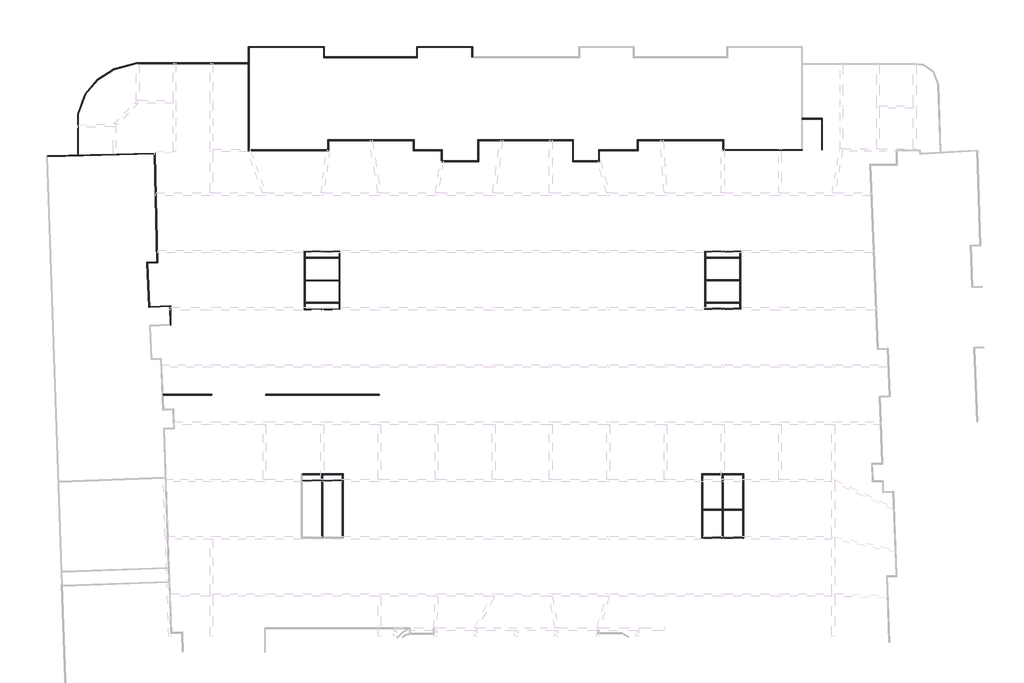
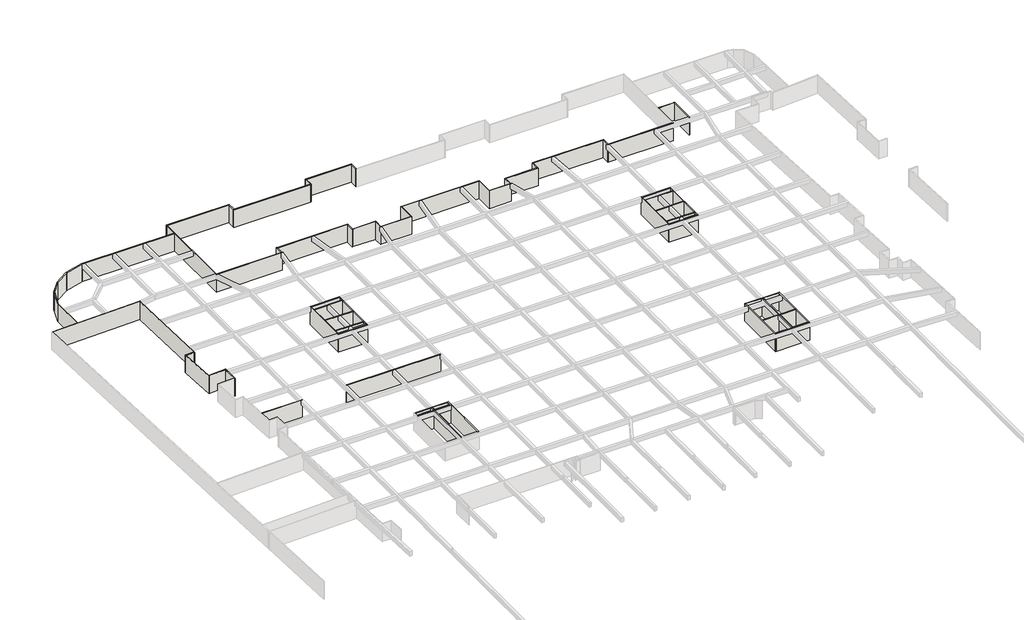
# One storey, part 3 of 8: 64 walls.
"""IFC4 building model written with IfcOpenShell, lengths in millimetres."""

from ifc_helpers import new_model, si_unit, origin, origin_with_axes, place, context, project, spatial, polyline, outline, extrude, faceted_brep, element, save

model = new_model("IFC4")

# Units and contexts
model_context = context("Model", 3, world=origin())
ifc_project = project(units=[si_unit("LENGTHUNIT", "METRE", prefix="MILLI")], contexts=[model_context])

# Site, building, storey
site = spatial("IfcSite", under=ifc_project)
building = spatial("IfcBuilding", under=site)
storey = spatial("IfcBuildingStorey", under=building, Name="户型图", Elevation=0.0)

# Walls
placement = place(None, origin())
element("IfcWall", 1, ObjectType="所有墙体", at=placement, inside=storey, context=model_context, shape_type="Brep", body=[
    faceted_brep([(652720.3094441, -903322.0093989, 0.0), (668403.5865909, -902923.6273505, 0.0), (668523.5478948, -902920.5801283, 0.0), (668523.5478948, -902920.5801283, 3300.0), (668403.5865909, -902923.6273505, 3300.0), (652720.3094441, -903322.0093989, 3300.0), (652716.1213151, -903202.077076, 0.0), (652716.1213151, -903202.077076, 3300.0), (657153.6402454, -903089.3565097, 3300.0), (657273.6402454, -903086.3083045, 3300.0), (668520.5006726, -902800.6188244, 3300.0), (668520.5006726, -902800.6188244, 0.0), (657273.6402454, -903086.3083045, 0.0), (657153.6402454, -903089.3565097, 0.0)], [[[0, 1, 2, 3, 4, 5]], [[6, 7, 8, 9, 10, 11, 12, 13]], [[2, 1, 0, 6, 13, 12, 11]], [[5, 4, 3, 10, 9, 8, 7]], [[0, 5, 7, 6]], [[3, 2, 11, 10]]]),
])
element("IfcWall", 2, ObjectType="所有墙体", at=placement, inside=storey, context=model_context, shape_type="Brep", body=[
    faceted_brep([(668403.5865909, -902923.6273505, 0.0), (668806.8356594, -918798.5065686, 0.0), (668809.8828816, -918918.4678725, 0.0), (668809.8828816, -918918.4678725, 3300.0), (668806.8356594, -918798.5065686, 3300.0), (668403.5865909, -902923.6273505, 3300.0), (668523.5478948, -902920.5801283, 0.0), (668523.5478948, -902920.5801283, 3300.0), (668929.8441855, -918915.4206503, 3300.0), (668929.8441855, -918915.4206503, 0.0)], [[[0, 1, 2, 3, 4, 5]], [[6, 7, 8, 9]], [[2, 1, 0, 6, 9]], [[5, 4, 3, 8, 7]], [[0, 5, 7, 6]], [[3, 2, 9, 8]]]),
])
element("IfcWall", 3, ObjectType="所有墙体", at=placement, inside=storey, context=model_context, shape_type="Brep", body=[
    faceted_brep([(668806.8356594, -918798.5065686, 0.0), (667306.1591427, -918836.6263174, 0.0), (667306.1591427, -918836.6263174, 3300.0), (668806.8356594, -918798.5065686, 3300.0), (668809.8828816, -918918.4678725, 0.0), (668809.8828816, -918918.4678725, 3300.0), (667431.4881043, -918953.4814561, 3300.0), (667311.504784, -918956.5292375, 3300.0), (667311.504784, -918956.5292375, 0.0), (667431.4881043, -918953.4814561, 0.0)], [[[0, 1, 2, 3]], [[4, 5, 6, 7, 8, 9]], [[1, 0, 4, 9, 8]], [[3, 2, 7, 6, 5]], [[0, 3, 5, 4]], [[2, 1, 8, 7]]]),
])
element("IfcWall", 4, ObjectType="所有墙体", at=placement, inside=storey, context=model_context, shape_type="Brep", body=[
    faceted_brep([(667311.504784, -918956.5292375, 0.0), (667601.6118634, -925463.6411151, 0.0), (667601.6118634, -925463.6411151, 3300.0), (667311.504784, -918956.5292375, 3300.0), (667431.4881043, -918953.4814561, 0.0), (667431.4881043, -918953.4814561, 3300.0), (667716.1481214, -925338.4155362, 3300.0), (667721.4927818, -925458.2964547, 3300.0), (667721.4927818, -925458.2964547, 0.0), (667716.1481214, -925338.4155362, 0.0)], [[[0, 1, 2, 3]], [[4, 5, 6, 7, 8, 9]], [[1, 0, 4, 9, 8]], [[3, 2, 7, 6, 5]], [[0, 3, 5, 4]], [[2, 1, 8, 7]]]),
])
element("IfcWall", 5, ObjectType="所有墙体", at=placement, inside=storey, context=model_context, shape_type="Brep", body=[
    faceted_brep([(667721.4927818, -925458.2964547, 0.0), (670697.0897488, -925325.6351816, 0.0), (670817.0147025, -925320.288558, 0.0), (670817.0147025, -925320.288558, 3300.0), (670697.0897488, -925325.6351816, 3300.0), (667721.4927818, -925458.2964547, 3300.0), (667716.1481214, -925338.4155362, 0.0), (667716.1481214, -925338.4155362, 3300.0), (670814.9196444, -925200.2627623, 3300.0), (670814.9196444, -925200.2627623, 0.0)], [[[0, 1, 2, 3, 4, 5]], [[6, 7, 8, 9]], [[2, 1, 0, 6, 9]], [[5, 4, 3, 8, 7]], [[0, 5, 7, 6]], [[3, 2, 9, 8]]]),
])
element("IfcWall", 6, ObjectType="所有墙体", at=placement, inside=storey, context=model_context, shape_type="Brep", body=[
    faceted_brep([(670697.0897488, -925325.6351816, 0.0), (670742.7384573, -927940.8479412, 0.0), (670744.8335153, -928060.8737369, 0.0), (670744.8335153, -928060.8737369, 3300.0), (670742.7384573, -927940.8479412, 3300.0), (670697.0897488, -925325.6351816, 3300.0), (670817.0147025, -925320.288558, 0.0), (670817.0147025, -925320.288558, 3300.0), (670864.758469, -928055.5271133, 3300.0), (670864.758469, -928055.5271133, 0.0)], [[[0, 1, 2, 3, 4, 5]], [[6, 7, 8, 9]], [[2, 1, 0, 6, 9]], [[5, 4, 3, 8, 7]], [[0, 5, 7, 6]], [[3, 2, 9, 8]]]),
])
element("IfcWall", 7, ObjectType="所有墙体", at=placement, inside=storey, context=model_context, shape_type="Brep", body=[
    faceted_brep([(766494.1555611, -902351.7569482, 0.0), (766494.1555611, -897691.7569482, 0.0), (766494.1555611, -897691.7569482, 3300.0), (766494.1555611, -902351.7569482, 3300.0), (766374.1555611, -902351.7569482, 0.0), (766374.1555611, -902351.7569482, 3300.0), (766374.1555611, -897811.7569482, 3300.0), (766374.1555611, -897691.7569482, 3300.0), (766374.1555611, -897691.7569482, 0.0), (766374.1555611, -897811.7569482, 0.0)], [[[0, 1, 2, 3]], [[4, 5, 6, 7, 8, 9]], [[1, 0, 4, 9, 8]], [[3, 2, 7, 6, 5]], [[0, 3, 5, 4]], [[2, 1, 8, 7]]]),
])
element("IfcWall", 8, ObjectType="所有墙体", at=placement, inside=storey, context=model_context, shape_type="SweptSolid", body=[
    extrude(outline(polyline([(763544.1555611, -897691.7569482), (766374.1555611, -897691.7569482), (766374.1555611, -897811.7569482), (763544.1555611, -897811.7569482), (763544.1555611, -897691.7569482)])), origin_with_axes(), (0.0, 0.0, 1.0), 3300.0),
])
element("IfcWall", 9, ObjectType="所有墙体", at=placement, inside=storey, context=model_context, shape_type="Brep", body=[
    faceted_brep([(715144.1555611, -888666.7569482, 0.0), (715144.1555611, -887166.8168633, 0.0), (715144.1555611, -887166.8168633, 3300.0), (715144.1555611, -888666.7569482, 3300.0), (715024.1555611, -888666.7569482, 0.0), (715024.1555611, -888666.7569482, 3300.0), (715024.1555611, -887286.8168633, 3300.0), (715024.1555611, -887166.8168633, 3300.0), (715024.1555611, -887166.8168633, 0.0), (715024.1555611, -887286.8168633, 0.0)], [[[0, 1, 2, 3]], [[4, 5, 6, 7, 8, 9]], [[1, 0, 4, 9, 8]], [[3, 2, 7, 6, 5]], [[0, 3, 5, 4]], [[2, 1, 8, 7]]]),
])
element("IfcWall", 10, ObjectType="所有墙体", at=placement, inside=storey, context=model_context, shape_type="Brep", body=[
    faceted_brep([(715024.1555611, -887166.8168633, 0.0), (706904.1555611, -887166.8168633, 0.0), (706904.1555611, -887166.8168633, 3300.0), (715024.1555611, -887166.8168633, 3300.0), (715024.1555611, -887286.8168633, 0.0), (715024.1555611, -887286.8168633, 3300.0), (707024.1555611, -887286.8168633, 3300.0), (706904.1555611, -887286.8168633, 3300.0), (706904.1555611, -887286.8168633, 0.0), (707024.1555611, -887286.8168633, 0.0)], [[[0, 1, 2, 3]], [[4, 5, 6, 7, 8, 9]], [[1, 0, 4, 9, 8]], [[3, 2, 7, 6, 5]], [[0, 3, 5, 4]], [[2, 1, 8, 7]]]),
])
element("IfcWall", 11, ObjectType="所有墙体", at=placement, inside=storey, context=model_context, shape_type="Brep", body=[
    faceted_brep([(706904.1555611, -887286.8168633, 0.0), (706904.1555611, -888666.7569482, 0.0), (706904.1555611, -888786.7569482, 0.0), (706904.1555611, -888786.7569482, 3300.0), (706904.1555611, -888666.7569482, 3300.0), (706904.1555611, -887286.8168633, 3300.0), (707024.1555611, -887286.8168633, 0.0), (707024.1555611, -887286.8168633, 3300.0), (707024.1555611, -888786.7569482, 3300.0), (707024.1555611, -888786.7569482, 0.0)], [[[0, 1, 2, 3, 4, 5]], [[6, 7, 8, 9]], [[2, 1, 0, 6, 9]], [[5, 4, 3, 8, 7]], [[0, 5, 7, 6]], [[3, 2, 9, 8]]]),
])
element("IfcWall", 12, ObjectType="所有墙体", at=placement, inside=storey, context=model_context, shape_type="Brep", body=[
    faceted_brep([(706904.1555611, -888666.7569482, 0.0), (693394.1555611, -888666.7569482, 0.0), (693274.1555611, -888666.7569482, 0.0), (693274.1555611, -888666.7569482, 3300.0), (693394.1555611, -888666.7569482, 3300.0), (706904.1555611, -888666.7569482, 3300.0), (706904.1555611, -888786.7569482, 0.0), (706904.1555611, -888786.7569482, 3300.0), (693274.1555611, -888786.7569482, 3300.0), (693274.1555611, -888786.7569482, 0.0)], [[[0, 1, 2, 3, 4, 5]], [[6, 7, 8, 9]], [[2, 1, 0, 6, 9]], [[5, 4, 3, 8, 7]], [[0, 5, 7, 6]], [[3, 2, 9, 8]]]),
])
element("IfcWall", 13, ObjectType="所有墙体", at=placement, inside=storey, context=model_context, shape_type="Brep", body=[
    faceted_brep([(693394.1555611, -888666.7569482, 0.0), (693394.1555611, -887166.8168633, 0.0), (693394.1555611, -887166.8168633, 3300.0), (693394.1555611, -888666.7569482, 3300.0), (693274.1555611, -888666.7569482, 0.0), (693274.1555611, -888666.7569482, 3300.0), (693274.1555611, -887286.8168633, 3300.0), (693274.1555611, -887166.8168633, 3300.0), (693274.1555611, -887166.8168633, 0.0), (693274.1555611, -887286.8168633, 0.0)], [[[0, 1, 2, 3]], [[4, 5, 6, 7, 8, 9]], [[1, 0, 4, 9, 8]], [[3, 2, 7, 6, 5]], [[0, 3, 5, 4]], [[2, 1, 8, 7]]]),
])
element("IfcWall", 14, ObjectType="所有墙体", at=placement, inside=storey, context=model_context, shape_type="Brep", body=[
    faceted_brep([(693274.1555611, -887166.8168633, 0.0), (682227.1185384, -887166.8168633, 0.0), (682227.1185384, -887166.8168633, 3300.0), (693274.1555611, -887166.8168633, 3300.0), (693274.1555611, -887286.8168633, 0.0), (693274.1555611, -887286.8168633, 3300.0), (682347.1185384, -887286.8168633, 3300.0), (682227.1185384, -887286.8168633, 3300.0), (682227.1185384, -887286.8168633, 0.0), (682347.1185384, -887286.8168633, 0.0)], [[[0, 1, 2, 3]], [[4, 5, 6, 7, 8, 9]], [[1, 0, 4, 9, 8]], [[3, 2, 7, 6, 5]], [[0, 3, 5, 4]], [[2, 1, 8, 7]]]),
])
element("IfcWall", 15, ObjectType="所有墙体", at=placement, inside=storey, context=model_context, shape_type="Brep", body=[
    faceted_brep([(682227.1185384, -887286.8168633, 0.0), (682227.1185384, -889568.8408137, 0.0), (682227.1185384, -889688.8408137, 0.0), (682227.1185384, -902461.3967018, 0.0), (682227.1185384, -902461.3967018, 3300.0), (682227.1185384, -889688.8408137, 3300.0), (682227.1185384, -889568.8408137, 3300.0), (682227.1185384, -887286.8168633, 3300.0), (682347.1185384, -887286.8168633, 0.0), (682347.1185384, -887286.8168633, 3300.0), (682347.1185384, -902341.3967018, 3300.0), (682347.1185384, -902461.3967018, 3300.0), (682347.1185384, -902461.3967018, 0.0), (682347.1185384, -902341.3967018, 0.0)], [[[0, 1, 2, 3, 4, 5, 6, 7]], [[8, 9, 10, 11, 12, 13]], [[3, 2, 1, 0, 8, 13, 12]], [[7, 6, 5, 4, 11, 10, 9]], [[0, 7, 9, 8]], [[4, 3, 12, 11]]]),
])
element("IfcWall", 16, ObjectType="所有墙体", at=placement, inside=storey, context=model_context, shape_type="Brep", body=[
    faceted_brep([(682347.1185384, -902461.3967018, 0.0), (693994.1555611, -902461.3967018, 0.0), (693994.1555611, -902461.3967018, 3300.0), (682347.1185384, -902461.3967018, 3300.0), (682347.1185384, -902341.3967018, 0.0), (682347.1185384, -902341.3967018, 3300.0), (693874.1555611, -902341.3967018, 3300.0), (693994.1555611, -902341.3967018, 3300.0), (693994.1555611, -902341.3967018, 0.0), (693874.1555611, -902341.3967018, 0.0)], [[[0, 1, 2, 3]], [[4, 5, 6, 7, 8, 9]], [[1, 0, 4, 9, 8]], [[3, 2, 7, 6, 5]], [[0, 3, 5, 4]], [[2, 1, 8, 7]]]),
])
element("IfcWall", 17, ObjectType="所有墙体", at=placement, inside=storey, context=model_context, shape_type="Brep", body=[
    faceted_brep([(693994.1555611, -902341.3967018, 0.0), (693994.1555611, -900986.7569482, 0.0), (693994.1555611, -900866.7569482, 0.0), (693994.1555611, -900866.7569482, 3300.0), (693994.1555611, -900986.7569482, 3300.0), (693994.1555611, -902341.3967018, 3300.0), (693874.1555611, -902341.3967018, 0.0), (693874.1555611, -902341.3967018, 3300.0), (693874.1555611, -900866.7569482, 3300.0), (693874.1555611, -900866.7569482, 0.0)], [[[0, 1, 2, 3, 4, 5]], [[6, 7, 8, 9]], [[2, 1, 0, 6, 9]], [[5, 4, 3, 8, 7]], [[0, 5, 7, 6]], [[3, 2, 9, 8]]]),
])
element("IfcWall", 18, ObjectType="所有墙体", at=placement, inside=storey, context=model_context, shape_type="Brep", body=[
    faceted_brep([(693994.1555611, -900986.7569482, 0.0), (706424.1555611, -900986.7569482, 0.0), (706544.1555611, -900986.7569482, 0.0), (706544.1555611, -900986.7569482, 3300.0), (706424.1555611, -900986.7569482, 3300.0), (693994.1555611, -900986.7569482, 3300.0), (693994.1555611, -900866.7569482, 0.0), (693994.1555611, -900866.7569482, 3300.0), (706544.1555611, -900866.7569482, 3300.0), (706544.1555611, -900866.7569482, 0.0)], [[[0, 1, 2, 3, 4, 5]], [[6, 7, 8, 9]], [[2, 1, 0, 6, 9]], [[5, 4, 3, 8, 7]], [[0, 5, 7, 6]], [[3, 2, 9, 8]]]),
])
element("IfcWall", 19, ObjectType="所有墙体", at=placement, inside=storey, context=model_context, shape_type="Brep", body=[
    faceted_brep([(706424.1555611, -900986.7569482, 0.0), (706424.1555611, -902461.3967018, 0.0), (706424.1555611, -902461.3967018, 3300.0), (706424.1555611, -900986.7569482, 3300.0), (706544.1555611, -900986.7569482, 0.0), (706544.1555611, -900986.7569482, 3300.0), (706544.1555611, -902341.3967018, 3300.0), (706544.1555611, -902461.3967018, 3300.0), (706544.1555611, -902461.3967018, 0.0), (706544.1555611, -902341.3967018, 0.0)], [[[0, 1, 2, 3]], [[4, 5, 6, 7, 8, 9]], [[1, 0, 4, 9, 8]], [[3, 2, 7, 6, 5]], [[0, 3, 5, 4]], [[2, 1, 8, 7]]]),
])
element("IfcWall", 20, ObjectType="所有墙体", at=placement, inside=storey, context=model_context, shape_type="Brep", body=[
    faceted_brep([(706544.1555611, -902461.3967018, 0.0), (710546.3042159, -902461.3967018, 0.0), (710666.3042159, -902461.3967018, 0.0), (710666.3042159, -902461.3967018, 3300.0), (710546.3042159, -902461.3967018, 3300.0), (706544.1555611, -902461.3967018, 3300.0), (706544.1555611, -902341.3967018, 0.0), (706544.1555611, -902341.3967018, 3300.0), (710666.3042159, -902341.3967018, 3300.0), (710666.3042159, -902341.3967018, 0.0)], [[[0, 1, 2, 3, 4, 5]], [[6, 7, 8, 9]], [[2, 1, 0, 6, 9]], [[5, 4, 3, 8, 7]], [[0, 5, 7, 6]], [[3, 2, 9, 8]]]),
])
element("IfcWall", 21, ObjectType="所有墙体", at=placement, inside=storey, context=model_context, shape_type="Brep", body=[
    faceted_brep([(710546.3042159, -902461.3967018, 0.0), (710546.3042159, -904061.7569482, 0.0), (710546.3042159, -904061.7569482, 3300.0), (710546.3042159, -902461.3967018, 3300.0), (710666.3042159, -902461.3967018, 0.0), (710666.3042159, -902461.3967018, 3300.0), (710666.3042159, -903941.7569482, 3300.0), (710666.3042159, -904061.7569482, 3300.0), (710666.3042159, -904061.7569482, 0.0), (710666.3042159, -903941.7569482, 0.0)], [[[0, 1, 2, 3]], [[4, 5, 6, 7, 8, 9]], [[1, 0, 4, 9, 8]], [[3, 2, 7, 6, 5]], [[0, 3, 5, 4]], [[2, 1, 8, 7]]]),
])
element("IfcWall", 22, ObjectType="所有墙体", at=placement, inside=storey, context=model_context, shape_type="Brep", body=[
    faceted_brep([(710666.3042159, -904061.7569482, 0.0), (716044.1555611, -904061.7569482, 0.0), (716044.1555611, -904061.7569482, 3300.0), (710666.3042159, -904061.7569482, 3300.0), (710666.3042159, -903941.7569482, 0.0), (710666.3042159, -903941.7569482, 3300.0), (715924.1555611, -903941.7569482, 3300.0), (716044.1555611, -903941.7569482, 3300.0), (716044.1555611, -903941.7569482, 0.0), (715924.1555611, -903941.7569482, 0.0)], [[[0, 1, 2, 3]], [[4, 5, 6, 7, 8, 9]], [[1, 0, 4, 9, 8]], [[3, 2, 7, 6, 5]], [[0, 3, 5, 4]], [[2, 1, 8, 7]]]),
])
element("IfcWall", 23, ObjectType="所有墙体", at=placement, inside=storey, context=model_context, shape_type="Brep", body=[
    faceted_brep([(716044.1555611, -903941.7569482, 0.0), (716044.1555611, -900986.7569482, 0.0), (716044.1555611, -900866.7569482, 0.0), (716044.1555611, -900866.7569482, 3300.0), (716044.1555611, -900986.7569482, 3300.0), (716044.1555611, -903941.7569482, 3300.0), (715924.1555611, -903941.7569482, 0.0), (715924.1555611, -903941.7569482, 3300.0), (715924.1555611, -900866.7569482, 3300.0), (715924.1555611, -900866.7569482, 0.0)], [[[0, 1, 2, 3, 4, 5]], [[6, 7, 8, 9]], [[2, 1, 0, 6, 9]], [[5, 4, 3, 8, 7]], [[0, 5, 7, 6]], [[3, 2, 9, 8]]]),
])
element("IfcWall", 24, ObjectType="所有墙体", at=placement, inside=storey, context=model_context, shape_type="Brep", body=[
    faceted_brep([(716044.1555611, -900986.7569482, 0.0), (729824.1555611, -900986.7569482, 0.0), (729944.1555611, -900986.7569482, 0.0), (729944.1555611, -900986.7569482, 3300.0), (729824.1555611, -900986.7569482, 3300.0), (716044.1555611, -900986.7569482, 3300.0), (716044.1555611, -900866.7569482, 0.0), (716044.1555611, -900866.7569482, 3300.0), (729944.1555611, -900866.7569482, 3300.0), (729944.1555611, -900866.7569482, 0.0)], [[[0, 1, 2, 3, 4, 5]], [[6, 7, 8, 9]], [[2, 1, 0, 6, 9]], [[5, 4, 3, 8, 7]], [[0, 5, 7, 6]], [[3, 2, 9, 8]]]),
])
element("IfcWall", 25, ObjectType="所有墙体", at=placement, inside=storey, context=model_context, shape_type="Brep", body=[
    faceted_brep([(729824.1555611, -900986.7569482, 0.0), (729824.1555611, -904061.7569482, 0.0), (729824.1555611, -904061.7569482, 3300.0), (729824.1555611, -900986.7569482, 3300.0), (729944.1555611, -900986.7569482, 0.0), (729944.1555611, -900986.7569482, 3300.0), (729944.1555611, -903941.7569482, 3300.0), (729944.1555611, -904061.7569482, 3300.0), (729944.1555611, -904061.7569482, 0.0), (729944.1555611, -903941.7569482, 0.0)], [[[0, 1, 2, 3]], [[4, 5, 6, 7, 8, 9]], [[1, 0, 4, 9, 8]], [[3, 2, 7, 6, 5]], [[0, 3, 5, 4]], [[2, 1, 8, 7]]]),
])
element("IfcWall", 26, ObjectType="所有墙体", at=placement, inside=storey, context=model_context, shape_type="Brep", body=[
    faceted_brep([(729944.1555611, -904061.7569482, 0.0), (733744.1555611, -904061.7569482, 0.0), (733744.1555611, -904061.7569482, 3300.0), (729944.1555611, -904061.7569482, 3300.0), (729944.1555611, -903941.7569482, 0.0), (729944.1555611, -903941.7569482, 3300.0), (733624.1555611, -903941.7569482, 3300.0), (733744.1555611, -903941.7569482, 3300.0), (733744.1555611, -903941.7569482, 0.0), (733624.1555611, -903941.7569482, 0.0)], [[[0, 1, 2, 3]], [[4, 5, 6, 7, 8, 9]], [[1, 0, 4, 9, 8]], [[3, 2, 7, 6, 5]], [[0, 3, 5, 4]], [[2, 1, 8, 7]]]),
])
element("IfcWall", 27, ObjectType="所有墙体", at=placement, inside=storey, context=model_context, shape_type="Brep", body=[
    faceted_brep([(733744.1555611, -903941.7569482, 0.0), (733744.1555611, -902461.3967018, 0.0), (733744.1555611, -902341.3967018, 0.0), (733744.1555611, -902341.3967018, 3300.0), (733744.1555611, -902461.3967018, 3300.0), (733744.1555611, -903941.7569482, 3300.0), (733624.1555611, -903941.7569482, 0.0), (733624.1555611, -903941.7569482, 3300.0), (733624.1555611, -902341.3967018, 3300.0), (733624.1555611, -902341.3967018, 0.0)], [[[0, 1, 2, 3, 4, 5]], [[6, 7, 8, 9]], [[2, 1, 0, 6, 9]], [[5, 4, 3, 8, 7]], [[0, 5, 7, 6]], [[3, 2, 9, 8]]]),
])
element("IfcWall", 28, ObjectType="所有墙体", at=placement, inside=storey, context=model_context, shape_type="Brep", body=[
    faceted_brep([(733744.1555611, -902461.3967018, 0.0), (739444.1555611, -902461.3967018, 0.0), (739444.1555611, -902461.3967018, 3300.0), (733744.1555611, -902461.3967018, 3300.0), (733744.1555611, -902341.3967018, 0.0), (733744.1555611, -902341.3967018, 3300.0), (739324.1555611, -902341.3967018, 3300.0), (739444.1555611, -902341.3967018, 3300.0), (739444.1555611, -902341.3967018, 0.0), (739324.1555611, -902341.3967018, 0.0)], [[[0, 1, 2, 3]], [[4, 5, 6, 7, 8, 9]], [[1, 0, 4, 9, 8]], [[3, 2, 7, 6, 5]], [[0, 3, 5, 4]], [[2, 1, 8, 7]]]),
])
element("IfcWall", 29, ObjectType="所有墙体", at=placement, inside=storey, context=model_context, shape_type="Brep", body=[
    faceted_brep([(739444.1555611, -902341.3967018, 0.0), (739444.1555611, -900986.7569482, 0.0), (739444.1555611, -900866.7569482, 0.0), (739444.1555611, -900866.7569482, 3300.0), (739444.1555611, -900986.7569482, 3300.0), (739444.1555611, -902341.3967018, 3300.0), (739324.1555611, -902341.3967018, 0.0), (739324.1555611, -902341.3967018, 3300.0), (739324.1555611, -900866.7569482, 3300.0), (739324.1555611, -900866.7569482, 0.0)], [[[0, 1, 2, 3, 4, 5]], [[6, 7, 8, 9]], [[2, 1, 0, 6, 9]], [[5, 4, 3, 8, 7]], [[0, 5, 7, 6]], [[3, 2, 9, 8]]]),
])
element("IfcWall", 30, ObjectType="所有墙体", at=placement, inside=storey, context=model_context, shape_type="Brep", body=[
    faceted_brep([(739444.1555611, -900986.7569482, 0.0), (751874.1555611, -900986.7569482, 0.0), (751994.1555611, -900986.7569482, 0.0), (751994.1555611, -900986.7569482, 3300.0), (751874.1555611, -900986.7569482, 3300.0), (739444.1555611, -900986.7569482, 3300.0), (739444.1555611, -900866.7569482, 0.0), (739444.1555611, -900866.7569482, 3300.0), (751994.1555611, -900866.7569482, 3300.0), (751994.1555611, -900866.7569482, 0.0)], [[[0, 1, 2, 3, 4, 5]], [[6, 7, 8, 9]], [[2, 1, 0, 6, 9]], [[5, 4, 3, 8, 7]], [[0, 5, 7, 6]], [[3, 2, 9, 8]]]),
])
element("IfcWall", 31, ObjectType="所有墙体", at=placement, inside=storey, context=model_context, shape_type="Brep", body=[
    faceted_brep([(751874.1555611, -900986.7569482, 0.0), (751874.1555611, -902411.7569482, 0.0), (751874.1555611, -902411.7569482, 3300.0), (751874.1555611, -900986.7569482, 3300.0), (751994.1555611, -900986.7569482, 0.0), (751994.1555611, -900986.7569482, 3300.0), (751994.1555611, -902291.7569482, 3300.0), (751994.1555611, -902411.7569482, 3300.0), (751994.1555611, -902411.7569482, 0.0), (751994.1555611, -902291.7569482, 0.0)], [[[0, 1, 2, 3]], [[4, 5, 6, 7, 8, 9]], [[1, 0, 4, 9, 8]], [[3, 2, 7, 6, 5]], [[0, 3, 5, 4]], [[2, 1, 8, 7]]]),
])
element("IfcWall", 32, ObjectType="所有墙体", at=placement, inside=storey, context=model_context, shape_type="Brep", body=[
    faceted_brep([(751994.1555611, -902411.7569482, 0.0), (763544.1555611, -902411.7569482, 0.0), (763544.1555611, -902411.7569482, 3300.0), (751994.1555611, -902411.7569482, 3300.0), (751994.1555611, -902291.7569482, 0.0), (751994.1555611, -902291.7569482, 3300.0), (763424.1555611, -902291.7569482, 3300.0), (763544.1555611, -902291.7569482, 3300.0), (763544.1555611, -902291.7569482, 0.0), (763424.1555611, -902291.7569482, 0.0)], [[[0, 1, 2, 3]], [[4, 5, 6, 7, 8, 9]], [[1, 0, 4, 9, 8]], [[3, 2, 7, 6, 5]], [[0, 3, 5, 4]], [[2, 1, 8, 7]]]),
])
element("IfcWall", 33, ObjectType="所有墙体", at=placement, inside=storey, context=model_context, shape_type="SweptSolid", body=[
    extrude(outline(polyline([(665779.2193885, -889568.8408137), (682227.1185384, -889568.8408137), (682227.1185384, -889688.8408137), (665795.0176882, -889688.8408137), (665779.2193885, -889568.8408137)])), origin_with_axes(), (0.0, 0.0, 1.0), 3300.0),
])
element("IfcWall", 34, ObjectType="所有墙体", at=placement, inside=storey, context=model_context, shape_type="SweptSolid", body=[
    extrude(outline(polyline([(662478.7800714, -890453.1908634), (665779.2193885, -889568.8408137), (665795.0176882, -889688.8408137), (662527.1613866, -890564.4602707), (662478.7800714, -890453.1908634)])), origin_with_axes(), (0.0, 0.0, 1.0), 3300.0),
])
element("IfcWall", 35, ObjectType="所有墙体", at=placement, inside=storey, context=model_context, shape_type="SweptSolid", body=[
    extrude(outline(polyline([(660003.7770369, -891999.7444055), (662478.7800714, -890453.1908634), (662527.1613866, -890564.4602707), (660083.4854634, -892091.4384611), (660003.7770369, -891999.7444055)])), origin_with_axes(), (0.0, 0.0, 1.0), 3300.0),
])
element("IfcWall", 36, ObjectType="所有墙体", at=placement, inside=storey, context=model_context, shape_type="Brep", body=[
    faceted_brep([(660003.7770369, -891999.7444055, 0.0), (658255.3415895, -894083.4486314, 0.0), (658255.3415895, -894083.4486314, 3300.0), (660003.7770369, -891999.7444055, 3300.0), (660083.4854634, -892091.4384611, 0.0), (660083.4854634, -892091.4384611, 3300.0), (658360.8678185, -894144.3742281, 3300.0), (658135.3415895, -894413.1459217, 3300.0), (658135.3415895, -894413.1459217, 0.0), (658360.8678185, -894144.3742281, 0.0)], [[[0, 1, 2, 3]], [[4, 5, 6, 7, 8, 9]], [[1, 0, 4, 9, 8]], [[3, 2, 7, 6, 5]], [[0, 3, 5, 4]], [[2, 1, 8, 7]]]),
])
element("IfcWall", 37, ObjectType="所有墙体", at=placement, inside=storey, context=model_context, shape_type="SweptSolid", body=[
    extrude(outline(polyline([(657153.6402454, -897110.3481974), (658135.3415895, -894413.1459217), (658360.8678185, -894144.3742281), (657273.6402454, -897131.5074351), (657153.6402454, -897110.3481974)])), origin_with_axes(), (0.0, 0.0, 1.0), 3300.0),
])
element("IfcWall", 38, ObjectType="所有墙体", at=placement, inside=storey, context=model_context, shape_type="SweptSolid", body=[
    extrude(outline(polyline([(657153.6402454, -903089.3565097), (657153.6402454, -897110.3481974), (657273.6402454, -897131.5074351), (657273.6402454, -903086.3083045), (657153.6402454, -903089.3565097)])), origin_with_axes(), (0.0, 0.0, 1.0), 3300.0),
])
element("IfcWall", 39, ObjectType="所有墙体", at=placement, inside=storey, context=model_context, shape_type="Brep", body=[
    faceted_brep([(690452.0478253, -917206.0928676, 0.0), (690452.0478253, -925826.0928676, 0.0), (690452.0478253, -925826.0928676, 3300.0), (690452.0478253, -917206.0928676, 3300.0), (690572.0478253, -917206.0928676, 0.0), (690572.0478253, -917206.0928676, 3300.0), (690572.0478253, -917326.0928676, 3300.0), (690572.0478253, -918106.0928676, 3300.0), (690572.0478253, -918226.0928676, 3300.0), (690572.0478253, -921456.0928676, 3300.0), (690572.0478253, -921576.0928676, 3300.0), (690572.0478253, -924706.0928676, 3300.0), (690572.0478253, -924826.0928676, 3300.0), (690572.0478253, -925706.0928676, 3300.0), (690572.0478253, -925826.0928676, 3300.0), (690572.0478253, -925826.0928676, 0.0), (690572.0478253, -925706.0928676, 0.0), (690572.0478253, -924826.0928676, 0.0), (690572.0478253, -924706.0928676, 0.0), (690572.0478253, -921576.0928676, 0.0), (690572.0478253, -921456.0928676, 0.0), (690572.0478253, -918226.0928676, 0.0), (690572.0478253, -918106.0928676, 0.0), (690572.0478253, -917326.0928676, 0.0)], [[[0, 1, 2, 3]], [[4, 5, 6, 7, 8, 9, 10, 11, 12, 13, 14, 15, 16, 17, 18, 19, 20, 21, 22, 23]], [[1, 0, 4, 23, 22, 21, 20, 19, 18, 17, 16, 15]], [[3, 2, 14, 13, 12, 11, 10, 9, 8, 7, 6, 5]], [[2, 1, 15, 14]], [[0, 3, 5, 4]]]),
])
element("IfcWall", 40, ObjectType="所有墙体", at=placement, inside=storey, context=model_context, shape_type="Brep", body=[
    faceted_brep([(690572.0478253, -925826.0928676, 0.0), (695672.0478253, -925826.0928676, 0.0), (695672.0478253, -925826.0928676, 3300.0), (690572.0478253, -925826.0928676, 3300.0), (690572.0478253, -925706.0928676, 0.0), (690572.0478253, -925706.0928676, 3300.0), (695552.0478253, -925706.0928676, 3300.0), (695672.0478253, -925706.0928676, 3300.0), (695672.0478253, -925706.0928676, 0.0), (695552.0478253, -925706.0928676, 0.0)], [[[0, 1, 2, 3]], [[4, 5, 6, 7, 8, 9]], [[1, 0, 4, 9, 8]], [[3, 2, 7, 6, 5]], [[0, 3, 5, 4]], [[2, 1, 8, 7]]]),
])
element("IfcWall", 41, ObjectType="所有墙体", at=placement, inside=storey, context=model_context, shape_type="Brep", body=[
    faceted_brep([(695672.0478253, -925706.0928676, 0.0), (695672.0478253, -917206.0928676, 0.0), (695672.0478253, -917206.0928676, 3300.0), (695672.0478253, -925706.0928676, 3300.0), (695552.0478253, -925706.0928676, 0.0), (695552.0478253, -925706.0928676, 3300.0), (695552.0478253, -924826.0928676, 3300.0), (695552.0478253, -924706.0928676, 3300.0), (695552.0478253, -921576.0928676, 3300.0), (695552.0478253, -921456.0928676, 3300.0), (695552.0478253, -918226.0928676, 3300.0), (695552.0478253, -918106.0928676, 3300.0), (695552.0478253, -917326.0928676, 3300.0), (695552.0478253, -917206.0928676, 3300.0), (695552.0478253, -917206.0928676, 0.0), (695552.0478253, -917326.0928676, 0.0), (695552.0478253, -918106.0928676, 0.0), (695552.0478253, -918226.0928676, 0.0), (695552.0478253, -921456.0928676, 0.0), (695552.0478253, -921576.0928676, 0.0), (695552.0478253, -924706.0928676, 0.0), (695552.0478253, -924826.0928676, 0.0)], [[[0, 1, 2, 3]], [[4, 5, 6, 7, 8, 9, 10, 11, 12, 13, 14, 15, 16, 17, 18, 19, 20, 21]], [[1, 0, 4, 21, 20, 19, 18, 17, 16, 15, 14]], [[3, 2, 13, 12, 11, 10, 9, 8, 7, 6, 5]], [[0, 3, 5, 4]], [[2, 1, 14, 13]]]),
])
element("IfcWall", 42, ObjectType="所有墙体", at=placement, inside=storey, context=model_context, shape_type="SweptSolid", body=[
    extrude(outline(polyline([(690572.0478253, -917206.0928676), (695552.0478253, -917206.0928676), (695552.0478253, -917326.0928676), (690572.0478253, -917326.0928676), (690572.0478253, -917206.0928676)])), origin_with_axes(), (0.0, 0.0, 1.0), 3300.0),
])
element("IfcWall", 43, ObjectType="所有墙体", at=placement, inside=storey, context=model_context, shape_type="SweptSolid", body=[
    extrude(outline(polyline([(695552.0478253, -918226.0928676), (690572.0478253, -918226.0928676), (690572.0478253, -918106.0928676), (695552.0478253, -918106.0928676), (695552.0478253, -918226.0928676)])), origin_with_axes(), (0.0, 0.0, 1.0), 3300.0),
])
element("IfcWall", 44, ObjectType="所有墙体", at=placement, inside=storey, context=model_context, shape_type="SweptSolid", body=[
    extrude(outline(polyline([(690572.0478253, -921456.0928676), (695552.0478253, -921456.0928676), (695552.0478253, -921576.0928676), (690572.0478253, -921576.0928676), (690572.0478253, -921456.0928676)])), origin_with_axes(), (0.0, 0.0, 1.0), 3300.0),
])
element("IfcWall", 45, ObjectType="所有墙体", at=placement, inside=storey, context=model_context, shape_type="SweptSolid", body=[
    extrude(outline(polyline([(695552.0478253, -924826.0928676), (690572.0478253, -924826.0928676), (690572.0478253, -924706.0928676), (695552.0478253, -924706.0928676), (695552.0478253, -924826.0928676)])), origin_with_axes(), (0.0, 0.0, 1.0), 3300.0),
])
element("IfcWall", 46, ObjectType="所有墙体", at=placement, inside=storey, context=model_context, shape_type="SweptSolid", body=[
    extrude(outline(polyline([(684762.0478253, -938204.4532802), (701462.0478253, -938204.4532802), (701462.0478253, -938324.4532802), (684762.0478253, -938324.4532802), (684762.0478253, -938204.4532802)])), origin_with_axes(), (0.0, 0.0, 1.0), 3300.0),
])
element("IfcWall", 47, ObjectType="所有墙体", at=placement, inside=storey, context=model_context, shape_type="SweptSolid", body=[
    extrude(outline(polyline([(676862.0478253, -938324.4532802), (669683.5281685, -938324.4532802), (669678.1781991, -938204.4532802), (676862.0478253, -938204.4532802), (676862.0478253, -938324.4532802)])), origin_with_axes(), (0.0, 0.0, 1.0), 3300.0),
])
element("IfcWall", 48, ObjectType="所有墙体", at=placement, inside=storey, context=model_context, shape_type="Brep", body=[
    faceted_brep([(696122.0478253, -959206.0928676, 0.0), (696122.0478253, -949906.0928676, 0.0), (696122.0478253, -949906.0928676, 3300.0), (696122.0478253, -959206.0928676, 3300.0), (696002.0478253, -959206.0928676, 0.0), (696002.0478253, -959206.0928676, 3300.0), (696002.0478253, -950926.0928676, 3300.0), (696002.0478253, -950806.0928676, 3300.0), (696002.0478253, -950026.0928676, 3300.0), (696002.0478253, -949906.0928676, 3300.0), (696002.0478253, -949906.0928676, 0.0), (696002.0478253, -950026.0928676, 0.0), (696002.0478253, -950806.0928676, 0.0), (696002.0478253, -950926.0928676, 0.0)], [[[0, 1, 2, 3]], [[4, 5, 6, 7, 8, 9, 10, 11, 12, 13]], [[1, 0, 4, 13, 12, 11, 10]], [[3, 2, 9, 8, 7, 6, 5]], [[0, 3, 5, 4]], [[2, 1, 10, 9]]]),
])
element("IfcWall", 49, ObjectType="所有墙体", at=placement, inside=storey, context=model_context, shape_type="Brep", body=[
    faceted_brep([(696002.0478253, -949906.0928676, 0.0), (690122.0478253, -949906.0928676, 0.0), (690122.0478253, -949906.0928676, 3300.0), (696002.0478253, -949906.0928676, 3300.0), (696002.0478253, -950026.0928676, 0.0), (696002.0478253, -950026.0928676, 3300.0), (693122.0478253, -950026.0928676, 3300.0), (693002.0478253, -950026.0928676, 3300.0), (690122.0478253, -950026.0928676, 3300.0), (690122.0478253, -950026.0928676, 0.0), (693002.0478253, -950026.0928676, 0.0), (693122.0478253, -950026.0928676, 0.0)], [[[0, 1, 2, 3]], [[4, 5, 6, 7, 8, 9, 10, 11]], [[1, 0, 4, 11, 10, 9]], [[3, 2, 8, 7, 6, 5]], [[2, 1, 9, 8]], [[0, 3, 5, 4]]]),
])
element("IfcWall", 50, ObjectType="所有墙体", at=placement, inside=storey, context=model_context, shape_type="Brep", body=[
    faceted_brep([(690122.0478253, -950926.0928676, 0.0), (693002.0478253, -950926.0928676, 0.0), (693122.0478253, -950926.0928676, 0.0), (696002.0478253, -950926.0928676, 0.0), (696002.0478253, -950926.0928676, 3300.0), (693122.0478253, -950926.0928676, 3300.0), (693002.0478253, -950926.0928676, 3300.0), (690122.0478253, -950926.0928676, 3300.0), (690122.0478253, -950806.0928676, 0.0), (690122.0478253, -950806.0928676, 3300.0), (693002.0478253, -950806.0928676, 3300.0), (693122.0478253, -950806.0928676, 3300.0), (696002.0478253, -950806.0928676, 3300.0), (696002.0478253, -950806.0928676, 0.0), (693122.0478253, -950806.0928676, 0.0), (693002.0478253, -950806.0928676, 0.0)], [[[0, 1, 2, 3, 4, 5, 6, 7]], [[8, 9, 10, 11, 12, 13, 14, 15]], [[3, 2, 1, 0, 8, 15, 14, 13]], [[7, 6, 5, 4, 12, 11, 10, 9]], [[4, 3, 13, 12]], [[0, 7, 9, 8]]]),
])
element("IfcWall", 51, ObjectType="所有墙体", at=placement, inside=storey, context=model_context, shape_type="SweptSolid", body=[
    extrude(outline(polyline([(693122.0478253, -959206.0928676), (693002.0478253, -959206.0928676), (693002.0478253, -950926.0928676), (693122.0478253, -950926.0928676), (693122.0478253, -959206.0928676)])), origin_with_axes(), (0.0, 0.0, 1.0), 3300.0),
    extrude(outline(polyline([(693002.0478253, -950026.0928676), (693122.0478253, -950026.0928676), (693122.0478253, -950806.0928676), (693002.0478253, -950806.0928676), (693002.0478253, -950026.0928676)])), origin_with_axes(), (0.0, 0.0, 1.0), 3300.0),
])
element("IfcWall", 52, ObjectType="所有墙体", at=placement, inside=storey, context=model_context, shape_type="Brep", body=[
    faceted_brep([(748802.0478253, -949906.0928676, 0.0), (748802.0478253, -959326.0928676, 0.0), (748802.0478253, -959326.0928676, 3300.0), (748802.0478253, -949906.0928676, 3300.0), (748922.0478253, -949906.0928676, 0.0), (748922.0478253, -949906.0928676, 3300.0), (748922.0478253, -950026.0928676, 3300.0), (748922.0478253, -955081.0928676, 3300.0), (748922.0478253, -955201.0928676, 3300.0), (748922.0478253, -959206.0928676, 3300.0), (748922.0478253, -959326.0928676, 3300.0), (748922.0478253, -959326.0928676, 0.0), (748922.0478253, -959206.0928676, 0.0), (748922.0478253, -955201.0928676, 0.0), (748922.0478253, -955081.0928676, 0.0), (748922.0478253, -950026.0928676, 0.0)], [[[0, 1, 2, 3]], [[4, 5, 6, 7, 8, 9, 10, 11, 12, 13, 14, 15]], [[1, 0, 4, 15, 14, 13, 12, 11]], [[3, 2, 10, 9, 8, 7, 6, 5]], [[2, 1, 11, 10]], [[0, 3, 5, 4]]]),
])
element("IfcWall", 53, ObjectType="所有墙体", at=placement, inside=storey, context=model_context, shape_type="Brep", body=[
    faceted_brep([(748922.0478253, -959326.0928676, 0.0), (754922.0478253, -959326.0928676, 0.0), (754922.0478253, -959326.0928676, 3300.0), (748922.0478253, -959326.0928676, 3300.0), (748922.0478253, -959206.0928676, 0.0), (748922.0478253, -959206.0928676, 3300.0), (751802.0478253, -959206.0928676, 3300.0), (751922.0478253, -959206.0928676, 3300.0), (754802.0478253, -959206.0928676, 3300.0), (754922.0478253, -959206.0928676, 3300.0), (754922.0478253, -959206.0928676, 0.0), (754802.0478253, -959206.0928676, 0.0), (751922.0478253, -959206.0928676, 0.0), (751802.0478253, -959206.0928676, 0.0)], [[[0, 1, 2, 3]], [[4, 5, 6, 7, 8, 9, 10, 11, 12, 13]], [[1, 0, 4, 13, 12, 11, 10]], [[3, 2, 9, 8, 7, 6, 5]], [[0, 3, 5, 4]], [[2, 1, 10, 9]]]),
])
element("IfcWall", 54, ObjectType="所有墙体", at=placement, inside=storey, context=model_context, shape_type="Brep", body=[
    faceted_brep([(754922.0478253, -959206.0928676, 0.0), (754922.0478253, -949906.0928676, 0.0), (754922.0478253, -949906.0928676, 3300.0), (754922.0478253, -959206.0928676, 3300.0), (754802.0478253, -959206.0928676, 0.0), (754802.0478253, -959206.0928676, 3300.0), (754802.0478253, -955201.0928676, 3300.0), (754802.0478253, -955081.0928676, 3300.0), (754802.0478253, -950026.0928676, 3300.0), (754802.0478253, -949906.0928676, 3300.0), (754802.0478253, -949906.0928676, 0.0), (754802.0478253, -950026.0928676, 0.0), (754802.0478253, -955081.0928676, 0.0), (754802.0478253, -955201.0928676, 0.0)], [[[0, 1, 2, 3]], [[4, 5, 6, 7, 8, 9, 10, 11, 12, 13]], [[1, 0, 4, 13, 12, 11, 10]], [[3, 2, 9, 8, 7, 6, 5]], [[0, 3, 5, 4]], [[2, 1, 10, 9]]]),
])
element("IfcWall", 55, ObjectType="所有墙体", at=placement, inside=storey, context=model_context, shape_type="Brep", body=[
    faceted_brep([(754802.0478253, -949906.0928676, 0.0), (748922.0478253, -949906.0928676, 0.0), (748922.0478253, -949906.0928676, 3300.0), (754802.0478253, -949906.0928676, 3300.0), (754802.0478253, -950026.0928676, 0.0), (754802.0478253, -950026.0928676, 3300.0), (751922.0478253, -950026.0928676, 3300.0), (751802.0478253, -950026.0928676, 3300.0), (748922.0478253, -950026.0928676, 3300.0), (748922.0478253, -950026.0928676, 0.0), (751802.0478253, -950026.0928676, 0.0), (751922.0478253, -950026.0928676, 0.0)], [[[0, 1, 2, 3]], [[4, 5, 6, 7, 8, 9, 10, 11]], [[1, 0, 4, 11, 10, 9]], [[3, 2, 8, 7, 6, 5]], [[2, 1, 9, 8]], [[0, 3, 5, 4]]]),
])
element("IfcWall", 56, ObjectType="所有墙体", at=placement, inside=storey, context=model_context, shape_type="Brep", body=[
    faceted_brep([(751802.0478253, -950026.0928676, 0.0), (751802.0478253, -955081.0928676, 0.0), (751802.0478253, -955201.0928676, 0.0), (751802.0478253, -959206.0928676, 0.0), (751802.0478253, -959206.0928676, 3300.0), (751802.0478253, -955201.0928676, 3300.0), (751802.0478253, -955081.0928676, 3300.0), (751802.0478253, -950026.0928676, 3300.0), (751922.0478253, -950026.0928676, 0.0), (751922.0478253, -950026.0928676, 3300.0), (751922.0478253, -955081.0928676, 3300.0), (751922.0478253, -955201.0928676, 3300.0), (751922.0478253, -959206.0928676, 3300.0), (751922.0478253, -959206.0928676, 0.0), (751922.0478253, -955201.0928676, 0.0), (751922.0478253, -955081.0928676, 0.0)], [[[0, 1, 2, 3, 4, 5, 6, 7]], [[8, 9, 10, 11, 12, 13, 14, 15]], [[3, 2, 1, 0, 8, 15, 14, 13]], [[7, 6, 5, 4, 12, 11, 10, 9]], [[4, 3, 13, 12]], [[0, 7, 9, 8]]]),
])
element("IfcWall", 57, ObjectType="所有墙体", at=placement, inside=storey, context=model_context, shape_type="SweptSolid", body=[
    extrude(outline(polyline([(748922.0478253, -955201.0928676), (748922.0478253, -955081.0928676), (751802.0478253, -955081.0928676), (751802.0478253, -955201.0928676), (748922.0478253, -955201.0928676)])), origin_with_axes(), (0.0, 0.0, 1.0), 3300.0),
    extrude(outline(polyline([(754802.0478253, -955081.0928676), (754802.0478253, -955201.0928676), (751922.0478253, -955201.0928676), (751922.0478253, -955081.0928676), (754802.0478253, -955081.0928676)])), origin_with_axes(), (0.0, 0.0, 1.0), 3300.0),
])
element("IfcWall", 58, ObjectType="所有墙体", at=placement, inside=storey, context=model_context, shape_type="Brep", body=[
    faceted_brep([(749252.0478253, -917206.0928676, 0.0), (749252.0478253, -925726.0928676, 0.0), (749252.0478253, -925726.0928676, 3300.0), (749252.0478253, -917206.0928676, 3300.0), (749372.0478253, -917206.0928676, 0.0), (749372.0478253, -917206.0928676, 3300.0), (749372.0478253, -917326.0928676, 3300.0), (749372.0478253, -918106.0928676, 3300.0), (749372.0478253, -918226.0928676, 3300.0), (749372.0478253, -921406.0928676, 3300.0), (749372.0478253, -921526.0928676, 3300.0), (749372.0478253, -924706.0928676, 3300.0), (749372.0478253, -924826.0928676, 3300.0), (749372.0478253, -925606.0928676, 3300.0), (749372.0478253, -925726.0928676, 3300.0), (749372.0478253, -925726.0928676, 0.0), (749372.0478253, -925606.0928676, 0.0), (749372.0478253, -924826.0928676, 0.0), (749372.0478253, -924706.0928676, 0.0), (749372.0478253, -921526.0928676, 0.0), (749372.0478253, -921406.0928676, 0.0), (749372.0478253, -918226.0928676, 0.0), (749372.0478253, -918106.0928676, 0.0), (749372.0478253, -917326.0928676, 0.0)], [[[0, 1, 2, 3]], [[4, 5, 6, 7, 8, 9, 10, 11, 12, 13, 14, 15, 16, 17, 18, 19, 20, 21, 22, 23]], [[1, 0, 4, 23, 22, 21, 20, 19, 18, 17, 16, 15]], [[3, 2, 14, 13, 12, 11, 10, 9, 8, 7, 6, 5]], [[2, 1, 15, 14]], [[0, 3, 5, 4]]]),
])
element("IfcWall", 59, ObjectType="所有墙体", at=placement, inside=storey, context=model_context, shape_type="Brep", body=[
    faceted_brep([(749372.0478253, -925726.0928676, 0.0), (754472.0478253, -925726.0928676, 0.0), (754472.0478253, -925726.0928676, 3300.0), (749372.0478253, -925726.0928676, 3300.0), (749372.0478253, -925606.0928676, 0.0), (749372.0478253, -925606.0928676, 3300.0), (754352.0478253, -925606.0928676, 3300.0), (754472.0478253, -925606.0928676, 3300.0), (754472.0478253, -925606.0928676, 0.0), (754352.0478253, -925606.0928676, 0.0)], [[[0, 1, 2, 3]], [[4, 5, 6, 7, 8, 9]], [[1, 0, 4, 9, 8]], [[3, 2, 7, 6, 5]], [[0, 3, 5, 4]], [[2, 1, 8, 7]]]),
])
element("IfcWall", 60, ObjectType="所有墙体", at=placement, inside=storey, context=model_context, shape_type="Brep", body=[
    faceted_brep([(754472.0478253, -925606.0928676, 0.0), (754472.0478253, -917206.0928676, 0.0), (754472.0478253, -917206.0928676, 3300.0), (754472.0478253, -925606.0928676, 3300.0), (754352.0478253, -925606.0928676, 0.0), (754352.0478253, -925606.0928676, 3300.0), (754352.0478253, -924826.0928676, 3300.0), (754352.0478253, -924706.0928676, 3300.0), (754352.0478253, -921526.0928676, 3300.0), (754352.0478253, -921406.0928676, 3300.0), (754352.0478253, -918226.0928676, 3300.0), (754352.0478253, -918106.0928676, 3300.0), (754352.0478253, -917326.0928676, 3300.0), (754352.0478253, -917206.0928676, 3300.0), (754352.0478253, -917206.0928676, 0.0), (754352.0478253, -917326.0928676, 0.0), (754352.0478253, -918106.0928676, 0.0), (754352.0478253, -918226.0928676, 0.0), (754352.0478253, -921406.0928676, 0.0), (754352.0478253, -921526.0928676, 0.0), (754352.0478253, -924706.0928676, 0.0), (754352.0478253, -924826.0928676, 0.0)], [[[0, 1, 2, 3]], [[4, 5, 6, 7, 8, 9, 10, 11, 12, 13, 14, 15, 16, 17, 18, 19, 20, 21]], [[1, 0, 4, 21, 20, 19, 18, 17, 16, 15, 14]], [[3, 2, 13, 12, 11, 10, 9, 8, 7, 6, 5]], [[0, 3, 5, 4]], [[2, 1, 14, 13]]]),
])
element("IfcWall", 61, ObjectType="所有墙体", at=placement, inside=storey, context=model_context, shape_type="SweptSolid", body=[
    extrude(outline(polyline([(749372.0478253, -917206.0928676), (754352.0478253, -917206.0928676), (754352.0478253, -917326.0928676), (749372.0478253, -917326.0928676), (749372.0478253, -917206.0928676)])), origin_with_axes(), (0.0, 0.0, 1.0), 3300.0),
])
element("IfcWall", 62, ObjectType="所有墙体", at=placement, inside=storey, context=model_context, shape_type="SweptSolid", body=[
    extrude(outline(polyline([(754352.0478253, -918226.0928676), (749372.0478253, -918226.0928676), (749372.0478253, -918106.0928676), (754352.0478253, -918106.0928676), (754352.0478253, -918226.0928676)])), origin_with_axes(), (0.0, 0.0, 1.0), 3300.0),
])
element("IfcWall", 63, ObjectType="所有墙体", at=placement, inside=storey, context=model_context, shape_type="SweptSolid", body=[
    extrude(outline(polyline([(749372.0478253, -921406.0928676), (754352.0478253, -921406.0928676), (754352.0478253, -921526.0928676), (749372.0478253, -921526.0928676), (749372.0478253, -921406.0928676)])), origin_with_axes(), (0.0, 0.0, 1.0), 3300.0),
])
element("IfcWall", 64, ObjectType="所有墙体", at=placement, inside=storey, context=model_context, shape_type="SweptSolid", body=[
    extrude(outline(polyline([(754352.0478253, -924826.0928676), (749372.0478253, -924826.0928676), (749372.0478253, -924706.0928676), (754352.0478253, -924706.0928676), (754352.0478253, -924826.0928676)])), origin_with_axes(), (0.0, 0.0, 1.0), 3300.0),
])

save(model, "model.ifc")

# Revit data of these elements
# Project information
#   项目发布日期 = "出图日期"
#   项目状态 = "项目状态"
#   客户姓名 = "所有者"
#   项目地址 = "## 街道\n省市自治区邮政编码"
#   项目名称 = "项目名称"
#   项目编号 = "项目编号"
# Type "所有墙体"
#   Layers, outside or top first: 120 mm "默认" (function 1)
# Elements 1, 2, 3, 4, 5, 6, 7, 8, 9, 10, 11, 12, 13, 14, 15, 16, 17, 18, 19, 20, 21, 22, 23, 24, 25, 26, 27, 28, 29, 30, 31, 32, 33, 34, 35, 36, 37, 38, 39, 40, 41, 42, 43, 44, 45, 46, 47, 48, 49, 50, 51, 52, 53, 54, 55, 56, 57, 58, 59, 60, 61, 62, 63, 64 (IfcWall, "所有墙体")
#   Top Offset = 0 mm
#   Base Offset = 0 mm
#   wall height = 3300 mm
#   Phase Created = 新构造
#   Base Constraint = 户型图
#   Top Constraint = 层高
#   Materials on its faces: "默认"
# Materials
#   "默认": class "其他", colour RGB 192 192 192, transparency 0, Cost = 0
# Area, not placed, upper offset 0 mm, lower offset 0 mm
#   Number = "165"
#   Name = "main_building"
# Area at (660629.431, -980851.65) mm, upper offset 0 mm, lower offset 0 mm
#   Number = "207"
#   Name = "main_building"
# Area at (763421.249, -980559.575) mm, upper offset 0 mm, lower offset 0 mm
#   Number = "215"
#   Name = "fire_compart"
# Area, not placed, upper offset 0 mm, lower offset 0 mm
#   Number = "80"
#   Name = "main_building"
# Area, not placed, upper offset 0 mm, lower offset 0 mm
#   Number = "118"
#   Name = "main_building"
# Area, not placed, upper offset 0 mm, lower offset 0 mm
#   Number = "160"
#   Name = "fire_compart"
# Area, not placed, upper offset 0 mm, lower offset 0 mm
#   Number = "149"
#   Name = "main_building"
# Area, not placed, upper offset 0 mm, lower offset 0 mm
#   Number = "182"
#   Name = "main_building"
# Area, not placed, upper offset 0 mm, lower offset 0 mm
#   Number = "81"
#   Name = "fire_compart"
# Area, not placed, upper offset 0 mm, lower offset 0 mm
#   Number = "82"
#   Name = "main_building"
# Area at (686527.876, -896584.337) mm, upper offset 0 mm, lower offset 0 mm
#   Number = "204"
#   Name = "main_building"
# Area, not placed, upper offset 0 mm, lower offset 0 mm
#   Number = "91"
#   Name = "main_building"
# Area, not placed, upper offset 0 mm, lower offset 0 mm
#   Number = "31"
#   Name = "main_building"
# Area, not placed, upper offset 0 mm, lower offset 0 mm
#   Number = "32"
#   Name = "main_building"
# Area, not placed, upper offset 0 mm, lower offset 0 mm
#   Number = "33"
#   Name = "main_building"
# Area, not placed, upper offset 0 mm, lower offset 0 mm
#   Number = "34"
#   Name = "main_building"
# Area, not placed, upper offset 0 mm, lower offset 0 mm
#   Number = "35"
#   Name = "main_building"
# Area, not placed, upper offset 0 mm, lower offset 0 mm
#   Number = "41"
#   Name = "main_building"
# Area, not placed, upper offset 0 mm, lower offset 0 mm
#   Number = "42"
#   Name = "main_building"
# Area, not placed, upper offset 0 mm, lower offset 0 mm
#   Number = "43"
#   Name = "main_building"
# Area, not placed, upper offset 0 mm, lower offset 0 mm
#   Number = "44"
#   Name = "main_building"
# Area, not placed, upper offset 0 mm, lower offset 0 mm
#   Number = "45"
#   Name = "main_building"
# Area, not placed, upper offset 0 mm, lower offset 0 mm
#   Number = "46"
#   Name = "main_building"
# Area, not placed, upper offset 0 mm, lower offset 0 mm
#   Number = "47"
#   Name = "main_building"
# Area, not placed, upper offset 0 mm, lower offset 0 mm
#   Number = "48"
#   Name = "main_building"
# Area, not placed, upper offset 0 mm, lower offset 0 mm
#   Number = "49"
#   Name = "main_building"
# Area, not placed, upper offset 0 mm, lower offset 0 mm
#   Number = "50"
#   Name = "main_building"
# Area, not placed, upper offset 0 mm, lower offset 0 mm
#   Number = "5"
#   Name = "fire_compart_3"
# Area, not placed, upper offset 0 mm, lower offset 0 mm
#   Number = "119"
#   Name = "main_building"
# Area, not placed, upper offset 0 mm, lower offset 0 mm
#   Number = "9"
#   Name = "main_building"
# Area, not placed, upper offset 0 mm, lower offset 0 mm
#   Number = "10"
#   Name = "main_building"
# Area, not placed, upper offset 0 mm, lower offset 0 mm
#   Number = "11"
#   Name = "main_building"
# Area, not placed, upper offset 0 mm, lower offset 0 mm
#   Number = "51"
#   Name = "fire_compart"
# Area, not placed, upper offset 0 mm, lower offset 0 mm
#   Number = "12"
#   Name = "main_building"
# Area, not placed, upper offset 0 mm, lower offset 0 mm
#   Number = "157"
#   Name = "fire_compart"
# Area, not placed, upper offset 0 mm, lower offset 0 mm
#   Number = "158"
#   Name = "fire_compart"
# Area, not placed, upper offset 0 mm, lower offset 0 mm
#   Number = "166"
#   Name = "main_building"
# Area, not placed, upper offset 0 mm, lower offset 0 mm
#   Number = "13"
#   Name = "main_building"
# Area, not placed, upper offset 0 mm, lower offset 0 mm
#   Number = "14"
#   Name = "main_building"
# Area, not placed, upper offset 0 mm, lower offset 0 mm
#   Number = "15"
#   Name = "main_building"
# Area, not placed, upper offset 0 mm, lower offset 0 mm
#   Number = "16"
#   Name = "main_building"
# Area, not placed, upper offset 0 mm, lower offset 0 mm
#   Number = "17"
#   Name = "main_building"
# Area, not placed, upper offset 0 mm, lower offset 0 mm
#   Number = "18"
#   Name = "main_building"
# Area, not placed, upper offset 0 mm, lower offset 0 mm
#   Number = "19"
#   Name = "面积"
# Area, not placed, upper offset 0 mm, lower offset 0 mm
#   Number = "20"
#   Name = "main_building"
# Area, not placed, upper offset 0 mm, lower offset 0 mm
#   Number = "21"
#   Name = "main_building"
# Area, not placed, upper offset 0 mm, lower offset 0 mm
#   Number = "22"
#   Name = "main_building"
# Area at (777372.745, -915011.014) mm, upper offset 0 mm, lower offset 0 mm
#   Number = "205"
#   Name = "main_building"
# Area, not placed, upper offset 0 mm, lower offset 0 mm
#   Number = "107"
#   Name = "main_building"
# Area, not placed, upper offset 0 mm, lower offset 0 mm
#   Number = "120"
#   Name = "main_building"
# Area, not placed, upper offset 0 mm, lower offset 0 mm
#   Number = "183"
#   Name = "main_building"
# Area, not placed, upper offset 0 mm, lower offset 0 mm
#   Number = "74"
#   Name = "main_building"
# Room, not placed, phase "新构造", upper offset 0 mm, lower offset 0 mm
#   Number = "9"
#   Name = "客餐厅轮廓"
# Area, not placed, upper offset 0 mm, lower offset 0 mm
#   Number = "92"
#   Name = "fire_compart"
# Area, not placed, upper offset 0 mm, lower offset 0 mm
#   Number = "93"
#   Name = "main_building"
# Area, not placed, upper offset 0 mm, lower offset 0 mm
#   Number = "94"
#   Name = "main_building"
# Room, not placed, phase "新构造", upper offset 0 mm, lower offset 0 mm
#   Number = "10"
#   Name = "墙面轮廓"
# Area, not placed, upper offset 0 mm, lower offset 0 mm
#   Number = "184"
#   Name = "main_building"
# Area, not placed, upper offset 0 mm, lower offset 0 mm
#   Number = "52"
#   Name = "fire_compart"
# Area, not placed, upper offset 0 mm, lower offset 0 mm
#   Number = "53"
#   Name = "fire_compart"
# Area, not placed, upper offset 0 mm, lower offset 0 mm
#   Number = "102"
#   Name = "main_building"
# Area, not placed, upper offset 0 mm, lower offset 0 mm
#   Number = "121"
#   Name = "main_building"
# Area, not placed, upper offset 0 mm, lower offset 0 mm
#   Number = "54"
#   Name = "fire_compart"
# Area at (711816.542, -1002868.718) mm, upper offset 0 mm, lower offset 0 mm
#   Number = "206"
#   Name = "main_building"
# Area, not placed, upper offset 0 mm, lower offset 0 mm
#   Number = "169"
#   Name = "main_building"
# Area, not placed, upper offset 0 mm, lower offset 0 mm
#   Number = "170"
#   Name = "fire_compart"
# Area, not placed, upper offset 0 mm, lower offset 0 mm
#   Number = "95"
#   Name = "fire_compart"
# Area, not placed, upper offset 0 mm, lower offset 0 mm
#   Number = "96"
#   Name = "main_building"
# Area, not placed, upper offset 0 mm, lower offset 0 mm
#   Number = "97"
#   Name = "main_building"
# Area, not placed, upper offset 0 mm, lower offset 0 mm
#   Number = "122"
#   Name = "main_building"
# Area, not placed, upper offset 0 mm, lower offset 0 mm
#   Number = "148"
#   Name = "main_building"
# Area, not placed, upper offset 0 mm, lower offset 0 mm
#   Number = "6"
#   Name = "fire_compart_4"
# Area, not placed, upper offset 0 mm, lower offset 0 mm
#   Number = "55"
#   Name = "fire_compart"
# Area, not placed, upper offset 0 mm, lower offset 0 mm
#   Number = "171"
#   Name = "fire_compart"
# Area, not placed, upper offset 0 mm, lower offset 0 mm
#   Number = "185"
#   Name = "main_building"
# Area, not placed, upper offset 0 mm, lower offset 0 mm
#   Number = "56"
#   Name = "fire_compart"
# Area, not placed, upper offset 0 mm, lower offset 0 mm
#   Number = "142"
#   Name = "fire_compart"
# Area, not placed, upper offset 0 mm, lower offset 0 mm
#   Number = "57"
#   Name = "fire_compart"
# Area, not placed, upper offset 0 mm, lower offset 0 mm
#   Number = "24"
#   Name = "fire_compart"
# Area, not placed, upper offset 0 mm, lower offset 0 mm
#   Number = "103"
#   Name = "main_building"
# Area, not placed, upper offset 0 mm, lower offset 0 mm
#   Number = "58"
#   Name = "fire_compart"
# Area, not placed, upper offset 0 mm, lower offset 0 mm
#   Number = "98"
#   Name = "fire_compart"
# Area, not placed, upper offset 0 mm, lower offset 0 mm
#   Number = "99"
#   Name = "main_building"
# Area, not placed, upper offset 0 mm, lower offset 0 mm
#   Number = "123"
#   Name = "main_building"
# Area, not placed, upper offset 0 mm, lower offset 0 mm
#   Number = "186"
#   Name = "main_building"
# Area at (660261.158, -937616.384) mm, upper offset 0 mm, lower offset 0 mm
#   Number = "208"
#   Name = "main_building"
# Area, not placed, upper offset 0 mm, lower offset 0 mm
#   Number = "209"
#   Name = "面积"
# Area, not placed, upper offset 0 mm, lower offset 0 mm
#   Number = "172"
#   Name = "fire_compart"
# Area, not placed, upper offset 0 mm, lower offset 0 mm
#   Number = "59"
#   Name = "fire_compart"
# Area, not placed, upper offset 0 mm, lower offset 0 mm
#   Number = "161"
#   Name = "main_building"
# Area, not placed, upper offset 0 mm, lower offset 0 mm
#   Number = "167"
#   Name = "main_building"
# Room, not placed, phase "新构造", upper offset 0 mm, lower offset 0 mm
#   Number = "1"
#   Name = "客餐厅"
# Room, not placed, phase "新构造", upper offset 0 mm, lower offset 0 mm
#   Number = "2"
#   Name = "阳台"
# Area at (769772.805, -1040660.096) mm, upper offset 0 mm, lower offset 0 mm
#   Number = "210"
#   Name = "main_building"
# Room, not placed, phase "新构造", upper offset 0 mm, lower offset 0 mm
#   Number = "3"
#   Name = "次卧"
# Room, not placed, phase "新构造", upper offset 0 mm, lower offset 0 mm
#   Number = "4"
#   Name = "厨房"
# Area, not placed, upper offset 0 mm, lower offset 0 mm
#   Number = "108"
#   Name = "main_building"
# Room, not placed, phase "新构造", upper offset 0 mm, lower offset 0 mm
#   Number = "5"
#   Name = "卫生间"
# Room, not placed, phase "新构造", upper offset 0 mm, lower offset 0 mm
#   Number = "6"
#   Name = "次卧"
# Room, not placed, phase "新构造", upper offset 0 mm, lower offset 0 mm
#   Number = "7"
#   Name = "主卧"
# Area, not placed, upper offset 0 mm, lower offset 0 mm
#   Number = "60"
#   Name = "fire_compart"
# Area, not placed, upper offset 0 mm, lower offset 0 mm
#   Number = "173"
#   Name = "面积"
# Area, not placed, upper offset 0 mm, lower offset 0 mm
#   Number = "174"
#   Name = "fire_compart"
# Area, not placed, upper offset 0 mm, lower offset 0 mm
#   Number = "23"
#   Name = "main_building"
# Area, not placed, upper offset 0 mm, lower offset 0 mm
#   Number = "124"
#   Name = "fire_compart"
# Area, not placed, upper offset 0 mm, lower offset 0 mm
#   Number = "36"
#   Name = "main_building"
# Area, not placed, upper offset 0 mm, lower offset 0 mm
#   Number = "37"
#   Name = "main_building"
# Area, not placed, upper offset 0 mm, lower offset 0 mm
#   Number = "38"
#   Name = "main_building"
# Area, not placed, upper offset 0 mm, lower offset 0 mm
#   Number = "39"
#   Name = "main_building"
# Area, not placed, upper offset 0 mm, lower offset 0 mm
#   Number = "40"
#   Name = "main_building"
